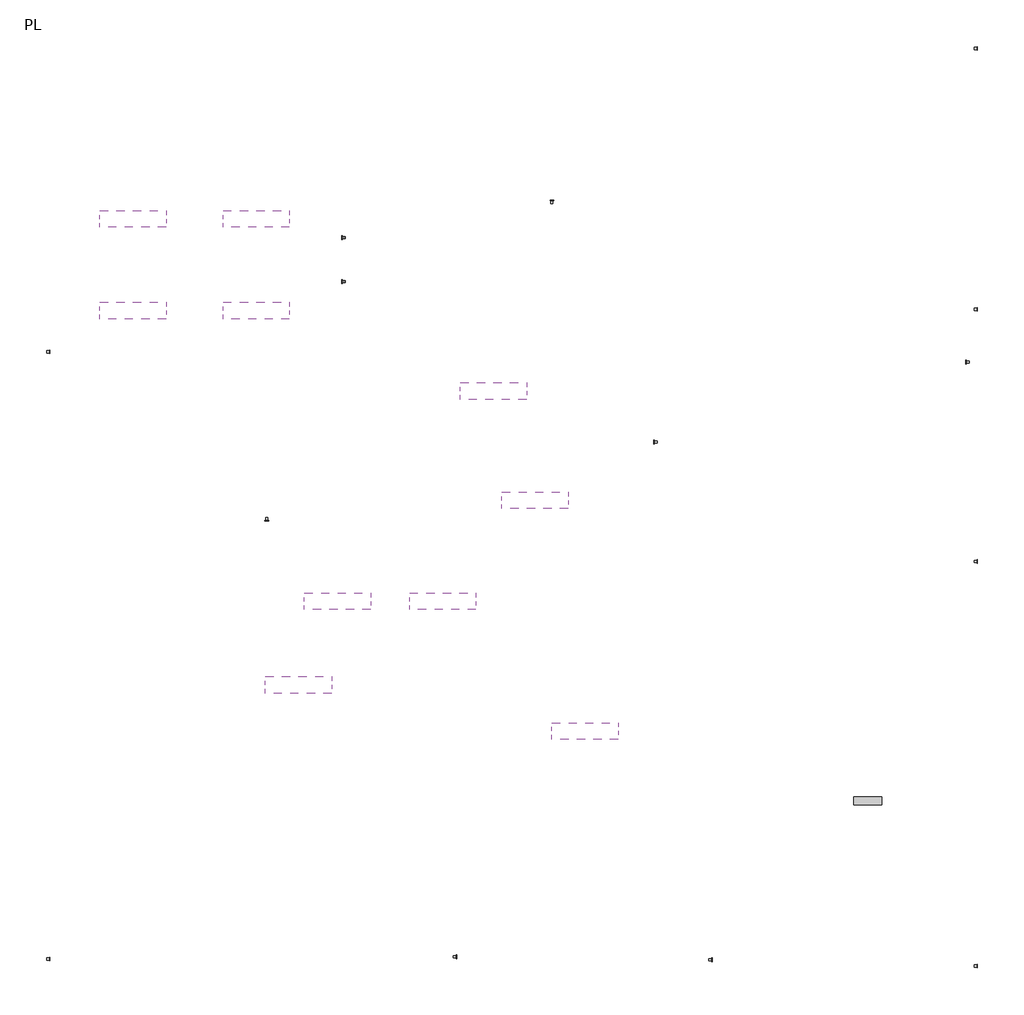
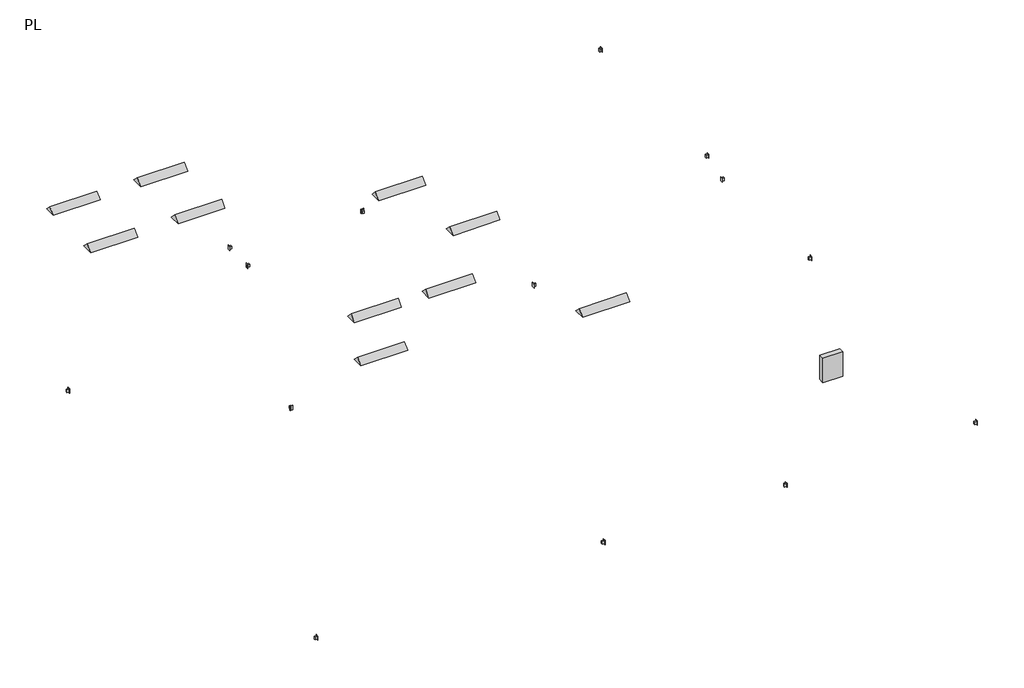
# One storey: 13 proxies, 10 light fixtures, 2 switching devices.
"""IFC4 building model written with IfcOpenShell, lengths in millimetres."""

import ifcopenshell
import ifcopenshell.guid

model = None  # the IFC model being written
_history = None  # IfcOwnerHistory: only IFC2X3 demands one
_inside = {}  # id of a spatial element -> (the spatial element, [elements in it])
_under = {}  # id of a project, library or spatial element -> (it, [spatial elements below it])
_declared = {}  # id of a project -> (the project, [libraries it declares])
_typed = {}  # id of a type object -> (the type object, [elements of that type])
_made_of = {}  # id of a material, layer set ... -> (it, [elements and type objects made of it])


def new_model(schema):
    """Start an empty IFC model of exactly this schema.

    Asked for "IFC4X3", IfcOpenShell would pick the latest addendum, in which some entities
    have other attributes; the version numbers below select the first issue.
    IFC2X3 requires an IfcOwnerHistory on every rooted entity: one is made here for all.
    """
    global model, _history
    if schema == "IFC4X3":
        model = ifcopenshell.file(schema_version=(4, 3, 0, 0))
    else:
        model = ifcopenshell.file(schema=schema)
    _inside.clear()
    _under.clear()
    _declared.clear()
    _typed.clear()
    _made_of.clear()
    _history = None
    if model.schema == "IFC2X3":
        org = make("IfcOrganization", Name="unknown")
        user = make(
            "IfcPersonAndOrganization",
            ThePerson=make("IfcPerson", FamilyName="unknown"),
            TheOrganization=org,
        )
        app = make(
            "IfcApplication",
            ApplicationDeveloper=org,
            Version="unknown",
            ApplicationFullName="unknown",
            ApplicationIdentifier="unknown",
        )
        _history = make(
            "IfcOwnerHistory",
            OwningUser=user,
            OwningApplication=app,
            ChangeAction="ADDED",
            CreationDate=0,
        )
    return model


def make(cls, **values):
    """One entity of the class cls with the attributes given. An attribute that is None is left unset."""
    return model.create_entity(
        cls, **{name: value for name, value in values.items() if value is not None}
    )


def rooted(cls, **values):
    """An entity with a GlobalId (a new one), such as an element, a storey or a relation."""
    return make(cls, GlobalId=ifcopenshell.guid.new(), OwnerHistory=_history, **values)


def si_unit(unit_type, name, prefix=None):
    """IfcSIUnit, for example si_unit("LENGTHUNIT", "METRE", prefix="MILLI")."""
    return make("IfcSIUnit", UnitType=unit_type, Prefix=prefix, Name=name)


def assignment(units):
    """IfcUnitAssignment: the units of a project."""
    return None if units is None else make("IfcUnitAssignment", Units=units)


def point(xyz):
    """IfcCartesianPoint."""
    return None if xyz is None else make("IfcCartesianPoint", Coordinates=xyz)


def direction(xyz):
    """IfcDirection."""
    return None if xyz is None else make("IfcDirection", DirectionRatios=xyz)


def frame(location, z_axis=None, x_axis=None):
    """IfcAxis2Placement3D, a coordinate frame: its origin and axes. An axis left out is left unset."""
    return make(
        "IfcAxis2Placement3D",
        Location=point(location),
        Axis=direction(z_axis),
        RefDirection=direction(x_axis),
    )


def origin():
    """The frame at (0, 0, 0) with its axes left unset."""
    return frame((0.0, 0.0, 0.0))


def origin_with_axes():
    """The frame at (0, 0, 0) with the z axis (0, 0, 1) and the x axis (1, 0, 0) written out."""
    return frame((0.0, 0.0, 0.0), z_axis=(0.0, 0.0, 1.0), x_axis=(1.0, 0.0, 0.0))


def place(relative_to, where):
    """IfcLocalPlacement: puts the frame where relative to a parent placement (None: the world)."""
    return make(
        "IfcLocalPlacement", PlacementRelTo=relative_to, RelativePlacement=where
    )


def context(
    kind, dimensions, precision=None, world=None, true_north=None, identifier=None
):
    """IfcGeometricRepresentationContext, for example the 3D "Model" context."""
    return make(
        "IfcGeometricRepresentationContext",
        ContextIdentifier=identifier,
        ContextType=kind,
        CoordinateSpaceDimension=dimensions,
        Precision=precision,
        WorldCoordinateSystem=world,
        TrueNorth=true_north,
    )


def project(units=None, contexts=None):
    """IfcProject with its units and contexts."""
    return rooted(
        "IfcProject",
        Name="project",
        RepresentationContexts=contexts,
        UnitsInContext=assignment(units),
    )


def spatial(cls, under=None, at=None, **own):
    """A site, building, storey or space (cls), placed at a placement, below another one or the project."""
    s = rooted(cls, ObjectPlacement=at, **own)
    if under is not None:
        _under.setdefault(under.id(), (under, []))[1].append(s)
    return s


def polyline(points):
    """IfcPolyline through the points."""
    return make("IfcPolyline", Points=[point(p) for p in points])


def outline(outer, holes=None, kind="AREA"):
    """IfcArbitraryClosedProfileDef: a profile drawn as a closed curve; with holes, ...WithVoids."""
    if holes is None:
        return make("IfcArbitraryClosedProfileDef", ProfileType=kind, OuterCurve=outer)
    return make(
        "IfcArbitraryProfileDefWithVoids",
        ProfileType=kind,
        OuterCurve=outer,
        InnerCurves=holes,
    )


def extrude(swept, where, along, depth):
    """IfcExtrudedAreaSolid: the profile swept, set in the frame where, extruded along a direction by depth."""
    return make(
        "IfcExtrudedAreaSolid",
        SweptArea=swept,
        Position=where,
        ExtrudedDirection=direction(along),
        Depth=depth,
    )


def shape(context_of_items, identifier, shape_type, items):
    """IfcShapeRepresentation: the items that make up one representation, for example the "Body"."""
    return make(
        "IfcShapeRepresentation",
        ContextOfItems=context_of_items,
        RepresentationIdentifier=identifier,
        RepresentationType=shape_type,
        Items=items,
    )


def source(mapping_origin, context_of_items, identifier, shape_type, items):
    """IfcRepresentationMap: a shape defined once, which mapped items show again and again."""
    return make(
        "IfcRepresentationMap",
        MappingOrigin=mapping_origin,
        MappedRepresentation=shape(context_of_items, identifier, shape_type, items),
    )


def transform(
    local_origin,
    x_axis=None,
    y_axis=None,
    z_axis=None,
    scale=None,
    scale2=None,
    scale3=None,
    uniform=True,
):
    """IfcCartesianTransformationOperator3D, or its non-uniform kind. x_axis, y_axis, z_axis: its Axis1, 2, 3."""
    if uniform:
        return make(
            "IfcCartesianTransformationOperator3D",
            Axis1=direction(x_axis),
            Axis2=direction(y_axis),
            LocalOrigin=point(local_origin),
            Scale=scale,
            Axis3=direction(z_axis),
        )
    return make(
        "IfcCartesianTransformationOperator3DnonUniform",
        Axis1=direction(x_axis),
        Axis2=direction(y_axis),
        LocalOrigin=point(local_origin),
        Scale=scale,
        Axis3=direction(z_axis),
        Scale2=scale2,
        Scale3=scale3,
    )


def mapped(mapping_source, mapping_target):
    """IfcMappedItem: shows the shape of a source again, moved by a transform."""
    return make(
        "IfcMappedItem", MappingSource=mapping_source, MappingTarget=mapping_target
    )


def made_of(thing, what):
    """Note that an element or type object is made of a material, layer set ...; save() writes the relation."""
    if what is not None:
        _made_of.setdefault(what.id(), (what, []))[1].append(thing)
    return thing


def element(
    cls,
    number,
    at=None,
    inside=None,
    cuts=None,
    type_object=None,
    material=None,
    context=None,
    identifier="Body",
    shape_type=None,
    held_by="IfcProductDefinitionShape",
    body=None,
    shapes=None,
    **own,
):
    """One element of the class cls, such as IfcWall. Its Tag is "e" and its number.

    at: its placement. inside: the storey or other place that contains it. cuts: it is an
    opening in that element (IfcRelVoidsElement). A single representation is given by context,
    identifier, shape_type and body (its items); several are given by shapes. held_by: the class
    of the entity that holds the representations. save() writes the other relations.
    """
    e = rooted(cls, Tag="e%d" % number, ObjectPlacement=at, **own)
    if body is not None:
        shapes = [shape(context, identifier, shape_type, body)]
    if shapes is not None:
        e.Representation = make(held_by, Representations=shapes)
    if inside is not None:
        _inside.setdefault(inside.id(), (inside, []))[1].append(e)
    if cuts is not None:
        rooted(
            "IfcRelVoidsElement", RelatingBuildingElement=cuts, RelatedOpeningElement=e
        )
    if type_object is not None:
        _typed.setdefault(type_object.id(), (type_object, []))[1].append(e)
    return made_of(e, material)


def aggregate(whole, parts):
    """IfcRelAggregates: a whole, such as a stair, and the parts it consists of."""
    return rooted("IfcRelAggregates", RelatingObject=whole, RelatedObjects=parts)


def save(model, path):
    """Write the relations noted so far, then the file.

    IfcRelAggregates (storeys below a building ...), IfcRelContainedInSpatialStructure (elements
    in a storey), IfcRelDefinesByType, IfcRelAssociatesMaterial and IfcRelDeclares: one each for
    every whole, place, type object, material and project.
    """
    for whole, parts in _under.values():
        aggregate(whole, parts)
    for where, things in _inside.values():
        rooted(
            "IfcRelContainedInSpatialStructure",
            RelatedElements=things,
            RelatingStructure=where,
        )
    for kind, things in _typed.values():
        rooted("IfcRelDefinesByType", RelatedObjects=things, RelatingType=kind)
    for what, things in _made_of.values():
        rooted("IfcRelAssociatesMaterial", RelatedObjects=things, RelatingMaterial=what)
    for by, libraries in _declared.values():
        rooted("IfcRelDeclares", RelatingContext=by, RelatedDefinitions=libraries)
    model.write(path)


def m_duplex_receptacle_standard_10251bba(model_context):
    return source(origin(), model_context, "Body", "SweptSolid", [
        extrude(outline(polyline([(19.05, 38.1), (19.05, -38.1), (-19.05, -38.1), (-19.05, 38.1), (19.05, 38.1)])), frame((0.0, 0.0, -53.975), z_axis=(0.0, 0.0, 1.0), x_axis=(1.0, 0.0, 0.0)), (0.0, 0.0, 1.0), 53.975),
        extrude(outline(polyline([(34.925, 57.15), (34.925, -57.15), (-34.925, -57.15), (-34.925, 57.15), (34.925, 57.15)])), origin_with_axes(), (0.0, 0.0, 1.0), 4.7625),
    ])


def m_lighting_and_appliance_panelboard_208v_mcb_100_a_975063b2(model_context):
    return source(origin(), model_context, "Body", "SweptSolid", [
        extrude(outline(polyline([(349.2594706, 94.0943297), (349.2594706, -566.3056703), (-158.7405294, -566.3056703), (-158.7405294, 94.0943297), (349.2594706, 94.0943297)])), frame((0.0, 0.0, -146.1), z_axis=(0.0, 0.0, 1.0), x_axis=(1.0, 0.0, 0.0)), (0.0, 0.0, 1.0), 146.1),
    ])


def m_plain_recessed_lighting_fixture_300x1200_120_e46e8774(model_context):
    return source(origin(), model_context, "Body", "SweptSolid", [
        extrude(outline(polyline([(-300.0, 0.0), (0.0, 0.0), (-150.0, -150.0), (-300.0, 0.0)])), frame((0.0, 0.0, 0.0), z_axis=(1.0, 0.0, 0.0), x_axis=(0.0, 1.0, 0.0)), (0.0, 0.0, 1.0), 1200.0),
    ])


model = new_model("IFC4")

# Units and contexts
model_context = context("Model", 3, world=origin())
ifc_project = project(units=[si_unit("LENGTHUNIT", "METRE", prefix="MILLI")], contexts=[model_context])

# Site, building, storey
site = spatial("IfcSite", under=ifc_project)
building = spatial("IfcBuilding", under=site)
storey = spatial("IfcBuildingStorey", under=building, Name="PL", Elevation=500.0)

# Proxies
placement = place(None, origin())
m_duplex_receptacle_standard_shape = m_duplex_receptacle_standard_10251bba(model_context)
element("IfcBuildingElementProxy", 1, Name="M_Duplex Receptacle : Standard", ObjectType="M_Duplex Receptacle : Standard", at=placement, inside=storey, context=model_context, shape_type="MappedRepresentation", body=[
    mapped(m_duplex_receptacle_standard_shape, transform((-14381.6781998, 2753.1971502, 960.0), x_axis=(0.0, -1.0, 0.0), y_axis=(0.0, 0.0, -1.0), z_axis=(1.0, 0.0, 0.0))),
])
element("IfcBuildingElementProxy", 2, Name="M_Duplex Receptacle : Standard", ObjectType="M_Duplex Receptacle : Standard", at=placement, inside=storey, context=model_context, shape_type="MappedRepresentation", body=[
    mapped(m_duplex_receptacle_standard_shape, transform((-14383.0803925, -8248.8260965, 945.9057387), x_axis=(0.0, -1.0, 0.0), y_axis=(0.0, 0.0, -1.0), z_axis=(1.0, 0.0, 0.0))),
])
element("IfcBuildingElementProxy", 3, Name="M_Duplex Receptacle : Standard", ObjectType="M_Duplex Receptacle : Standard", at=placement, inside=storey, context=model_context, shape_type="MappedRepresentation", body=[
    mapped(m_duplex_receptacle_standard_shape, transform((-7014.1011176, -8210.0342024, 931.5557962), x_axis=(0.0, -1.0, 0.0), y_axis=(0.0, 0.0, -1.0), z_axis=(1.0, 0.0, 0.0))),
])
element("IfcBuildingElementProxy", 4, Name="M_Duplex Receptacle : Standard", ObjectType="M_Duplex Receptacle : Standard", at=placement, inside=storey, context=model_context, shape_type="MappedRepresentation", body=[
    mapped(m_duplex_receptacle_standard_shape, transform((-2388.319764, -8264.9137548, 893.2417419), x_axis=(0.0, -1.0, 0.0), y_axis=(0.0, 0.0, -1.0), z_axis=(1.0, 0.0, 0.0))),
])
element("IfcBuildingElementProxy", 5, Name="M_Duplex Receptacle : Standard", ObjectType="M_Duplex Receptacle : Standard", at=placement, inside=storey, context=model_context, shape_type="MappedRepresentation", body=[
    mapped(m_duplex_receptacle_standard_shape, transform((2418.3218002, -8376.2820475, 960.0), x_axis=(0.0, -1.0, 0.0), y_axis=(0.0, 0.0, -1.0), z_axis=(1.0, 0.0, 0.0))),
])
element("IfcBuildingElementProxy", 6, Name="M_Duplex Receptacle : Standard", ObjectType="M_Duplex Receptacle : Standard", at=placement, inside=storey, context=model_context, shape_type="MappedRepresentation", body=[
    mapped(m_duplex_receptacle_standard_shape, transform((2418.3218002, -1043.6002542, 960.0), x_axis=(0.0, -1.0, 0.0), y_axis=(0.0, 0.0, -1.0), z_axis=(1.0, 0.0, 0.0))),
])
element("IfcBuildingElementProxy", 7, Name="M_Duplex Receptacle : Standard", ObjectType="M_Duplex Receptacle : Standard", at=placement, inside=storey, context=model_context, shape_type="MappedRepresentation", body=[
    mapped(m_duplex_receptacle_standard_shape, transform((2418.3218002, 3524.2201594, 960.0), x_axis=(0.0, -1.0, 0.0), y_axis=(0.0, 0.0, -1.0), z_axis=(1.0, 0.0, 0.0))),
])
element("IfcBuildingElementProxy", 8, Name="M_Duplex Receptacle : Standard", ObjectType="M_Duplex Receptacle : Standard", at=placement, inside=storey, context=model_context, shape_type="MappedRepresentation", body=[
    mapped(m_duplex_receptacle_standard_shape, transform((2418.3218002, 8251.436308, 960.0), x_axis=(0.0, -1.0, 0.0), y_axis=(0.0, 0.0, -1.0), z_axis=(1.0, 0.0, 0.0))),
])
element("IfcBuildingElementProxy", 9, Name="M_Duplex Receptacle : Standard", ObjectType="M_Duplex Receptacle : Standard", at=placement, inside=storey, context=model_context, shape_type="MappedRepresentation", body=[
    mapped(m_duplex_receptacle_standard_shape, transform((2218.3218002, 2571.4479124, 960.0), x_axis=(0.0, 1.0, 0.0), y_axis=(0.0, 0.0, -1.0), z_axis=(-1.0, 0.0, 0.0))),
])
element("IfcBuildingElementProxy", 10, Name="M_Duplex Receptacle : Standard", ObjectType="M_Duplex Receptacle : Standard", at=placement, inside=storey, context=model_context, shape_type="MappedRepresentation", body=[
    mapped(m_duplex_receptacle_standard_shape, transform((-5283.4743656, 5494.1412672, 960.0), x_axis=(1.0, 0.0, 0.0), y_axis=(0.0, 0.0, -1.0), z_axis=(0.0, 1.0, 0.0))),
])
element("IfcBuildingElementProxy", 11, Name="M_Duplex Receptacle : Standard", ObjectType="M_Duplex Receptacle : Standard", at=placement, inside=storey, context=model_context, shape_type="MappedRepresentation", body=[
    mapped(m_duplex_receptacle_standard_shape, transform((-10450.4315513, -305.8587328, 960.0), x_axis=(-1.0, 0.0, 0.0), y_axis=(0.0, 0.0, -1.0), z_axis=(0.0, -1.0, 0.0))),
])
element("IfcBuildingElementProxy", 12, Name="M_Duplex Receptacle : Standard", ObjectType="M_Duplex Receptacle : Standard", at=placement, inside=storey, context=model_context, shape_type="MappedRepresentation", body=[
    mapped(m_duplex_receptacle_standard_shape, transform((-3431.6781998, 1122.565095, 960.0), x_axis=(0.0, 1.0, 0.0), y_axis=(0.0, 0.0, -1.0), z_axis=(-1.0, 0.0, 0.0))),
])
m_lighting_and_appliance_panelboard_208v_mcb_100_a_shape = m_lighting_and_appliance_panelboard_208v_mcb_100_a_975063b2(model_context)
element("IfcBuildingElementProxy", 13, Name="M_Lighting and Appliance Panelboard - 208V MCB : 100 A", ObjectType="M_Lighting and Appliance Panelboard - 208V MCB : 100 A", at=placement, inside=storey, context=model_context, shape_type="MappedRepresentation", body=[
    mapped(m_lighting_and_appliance_panelboard_208v_mcb_100_a_shape, transform((337.9433717, -5451.9587328, 1605.9056703), x_axis=(1.0, 0.0, 0.0), y_axis=(0.0, 0.0, 1.0), z_axis=(0.0, -1.0, 0.0))),
])

# Light fixtures
m_plain_recessed_lighting_fixture_300x1200_120_shape = m_plain_recessed_lighting_fixture_300x1200_120_e46e8774(model_context)
element("IfcLightFixture", 14, ObjectType="M_Plain Recessed Lighting Fixture : 300x1200 - 120", at=placement, inside=storey, context=model_context, shape_type="MappedRepresentation", body=[
    mapped(m_plain_recessed_lighting_fixture_300x1200_120_shape, transform((-13471.5716878, 3351.0879554, 4000.0), x_axis=(1.0, 0.0, 0.0), y_axis=(0.0, -1.0, 0.0), z_axis=(0.0, 0.0, -1.0))),
])
element("IfcLightFixture", 15, ObjectType="M_Plain Recessed Lighting Fixture : 300x1200 - 120", at=placement, inside=storey, context=model_context, shape_type="MappedRepresentation", body=[
    mapped(m_plain_recessed_lighting_fixture_300x1200_120_shape, transform((-13471.5716878, 5008.8069678, 4000.0), x_axis=(1.0, 0.0, 0.0), y_axis=(0.0, -1.0, 0.0), z_axis=(0.0, 0.0, -1.0))),
])
element("IfcLightFixture", 16, ObjectType="M_Plain Recessed Lighting Fixture : 300x1200 - 120", at=placement, inside=storey, context=model_context, shape_type="MappedRepresentation", body=[
    mapped(m_plain_recessed_lighting_fixture_300x1200_120_shape, transform((-11238.106009, 5008.8069678, 4000.0), x_axis=(1.0, 0.0, 0.0), y_axis=(0.0, -1.0, 0.0), z_axis=(0.0, 0.0, -1.0))),
])
element("IfcLightFixture", 17, ObjectType="M_Plain Recessed Lighting Fixture : 300x1200 - 120", at=placement, inside=storey, context=model_context, shape_type="MappedRepresentation", body=[
    mapped(m_plain_recessed_lighting_fixture_300x1200_120_shape, transform((-11238.106009, 3351.0879554, 4000.0), x_axis=(1.0, 0.0, 0.0), y_axis=(0.0, -1.0, 0.0), z_axis=(0.0, 0.0, -1.0))),
])
element("IfcLightFixture", 18, ObjectType="M_Plain Recessed Lighting Fixture : 300x1200 - 120", at=placement, inside=storey, context=model_context, shape_type="MappedRepresentation", body=[
    mapped(m_plain_recessed_lighting_fixture_300x1200_120_shape, transform((-10474.940669, -3432.5980118, 4000.0), x_axis=(1.0, 0.0, 0.0), y_axis=(0.0, -1.0, 0.0), z_axis=(0.0, 0.0, -1.0))),
])
element("IfcLightFixture", 19, ObjectType="M_Plain Recessed Lighting Fixture : 300x1200 - 120", at=placement, inside=storey, context=model_context, shape_type="MappedRepresentation", body=[
    mapped(m_plain_recessed_lighting_fixture_300x1200_120_shape, transform((-5283.4493688, -4265.8003192, 4000.0), x_axis=(1.0, 0.0, 0.0), y_axis=(0.0, -1.0, 0.0), z_axis=(0.0, 0.0, -1.0))),
])
element("IfcLightFixture", 20, ObjectType="M_Plain Recessed Lighting Fixture : 300x1200 - 120", at=placement, inside=storey, context=model_context, shape_type="MappedRepresentation", body=[
    mapped(m_plain_recessed_lighting_fixture_300x1200_120_shape, transform((-6188.4168093, -89.5432203, 4000.0), x_axis=(1.0, 0.0, 0.0), y_axis=(0.0, -1.0, 0.0), z_axis=(0.0, 0.0, -1.0))),
])
element("IfcLightFixture", 21, ObjectType="M_Plain Recessed Lighting Fixture : 300x1200 - 120", at=placement, inside=storey, context=model_context, shape_type="MappedRepresentation", body=[
    mapped(m_plain_recessed_lighting_fixture_300x1200_120_shape, transform((-6944.285007, 1892.7111009, 4000.0), x_axis=(1.0, 0.0, 0.0), y_axis=(0.0, -1.0, 0.0), z_axis=(0.0, 0.0, -1.0))),
])
element("IfcLightFixture", 22, ObjectType="M_Plain Recessed Lighting Fixture : 300x1200 - 120", at=placement, inside=storey, context=model_context, shape_type="MappedRepresentation", body=[
    mapped(m_plain_recessed_lighting_fixture_300x1200_120_shape, transform((-7860.4121676, -1918.3778872, 4000.0), x_axis=(1.0, 0.0, 0.0), y_axis=(0.0, -1.0, 0.0), z_axis=(0.0, 0.0, -1.0))),
])
element("IfcLightFixture", 23, ObjectType="M_Plain Recessed Lighting Fixture : 300x1200 - 120", at=placement, inside=storey, context=model_context, shape_type="MappedRepresentation", body=[
    mapped(m_plain_recessed_lighting_fixture_300x1200_120_shape, transform((-9765.9566616, -1918.3778872, 4000.0), x_axis=(1.0, 0.0, 0.0), y_axis=(0.0, -1.0, 0.0), z_axis=(0.0, 0.0, -1.0))),
])

# Switching devices
element("IfcSwitchingDevice", 24, ObjectType="M_Lighting Switches : Three Way", at=placement, inside=storey, context=model_context, shape_type="MappedRepresentation", body=[
    mapped(m_duplex_receptacle_standard_shape, transform((-9081.6781998, 4824.0225299, 1700.0), x_axis=(0.0, -1.0, 0.0), y_axis=(0.0, 0.0, 1.0), z_axis=(-1.0, 0.0, 0.0))),
])
element("IfcSwitchingDevice", 25, ObjectType="M_Lighting Switches : Three Way", at=placement, inside=storey, context=model_context, shape_type="MappedRepresentation", body=[
    mapped(m_duplex_receptacle_standard_shape, transform((-9081.6781998, 4027.3902163, 1700.0), x_axis=(0.0, -1.0, 0.0), y_axis=(0.0, 0.0, 1.0), z_axis=(-1.0, 0.0, 0.0))),
])

save(model, "model.ifc")

# Revit data of these elements
# Project information
#   Project Issue Date = "Issue Date"
#   Project Status = "Project Status"
#   Client Name = "Owner"
#   Project Address = "Enter address here"
#   Project Name = "Project Name"
#   Project Number = "Project Number"
# Type "M_Duplex Receptacle : Standard"
#   Label = ""
#   Switch Voltage = 120 V
#   Load = 180 VA
#   Default Elevation = 460 mm
#   Load Classification = Receptacle
#   Assembly Code = ""
# Type "M_Lighting and Appliance Panelboard - 208V MCB : 100 A"
#   built-in parameter 1140081 [instance default] = "Recessed"
#   built-in parameter 1140083 [instance default] = "Type 1"
#   Width = 508 mm
#   built-in parameter 1140082 [instance default] = 100 (stored number, unit not read)
#   built-in parameter 1140140 = 100 (stored number, unit not read)
#   Height [instance default] = 584.2 mm
#   Depth = 146.1 mm
#   Default Elevation = 1200 mm
#   42 Circuit Height = 1270 mm
#   30 Circuit Height = 736.6 mm
#   24 Circuit Height = 660.4 mm
#   12 Circuit Height = 584.2 mm
#   built-in parameter 1140079 [instance default] = 12
#   Load Classification = Other
# Type "M_Plain Recessed Lighting Fixture : 300x1200 - 120"
#   Photometric Web File = "1x42A12.ies"
#   Width = 300 mm
#   Wattage = 64 W
#   built-in parameter 1150110 = 1 (stored number, unit not read)
#   built-in parameter 1150109 = 1 (stored number, unit not read)
#   built-in parameter 1150113 = 1 (stored number, unit not read)
#   Tilt Angle = -90.00°
#   Lumens = 5699.84 lm
#   built-in parameter 1114217 = 0.88 (stored number, unit not read)
#   built-in parameter 1150115 = 1 (stored number, unit not read)
#   built-in parameter 1150105 = 453.579 (stored number, unit not read)
#   Length = 1200 mm
#   built-in parameter 1150112 = 1 (stored number, unit not read)
#   built-in parameter 1150114 = 1 (stored number, unit not read)
#   built-in parameter 1150107 = 4230 (stored number, unit not read)
#   built-in parameter 1150106 = 4.53579 (stored number, unit not read)
#   Emit from Rectangle Width = 300 mm
#   Emit from Rectangle Length = 1200 mm
#   built-in parameter 1150104 = 8.27394 (stored number, unit not read)
#   Depth = 150 mm
#   Default Elevation = 2000 mm
#   Ballast Voltage = 120 V
#   built-in parameter 1114218 = 0.88 (stored number, unit not read)
#   built-in parameter 1150133 = 10 (stored number, unit not read)
#   Apparent Load = 64 VA
#   built-in parameter 1150134 = 8
#   built-in parameter 1150137 = 1
#   Color Filter = 16777215
#   built-in parameter 1140040 [instance default] = 1
#   Load Classification = Lighting - Dwelling Unit
#   Emit Shape Visible in Rendering = no
#   Dimming Lamp Color Temperature Shift = (empty or 0)
#   Assembly Code = ""
# Type "M_Lighting Switches : Three Way"
#   Label = "3"
#   Switch Voltage [instance default] = 120 V
#   Default Elevation = 1200 mm
#   Apparent Load = 0 VA
#   Load Classification = Other
#   Assembly Code = ""
# Element 1 (IfcBuildingElementProxy, "M_Duplex Receptacle : Standard")
#   Mark = "1"
#   Phase Created = New Construction
# Element 2 (IfcBuildingElementProxy, "M_Duplex Receptacle : Standard")
#   Mark = "2"
#   Phase Created = New Construction
# Element 3 (IfcBuildingElementProxy, "M_Duplex Receptacle : Standard")
#   Mark = "3"
#   Phase Created = New Construction
# Element 4 (IfcBuildingElementProxy, "M_Duplex Receptacle : Standard")
#   Mark = "4"
#   Phase Created = New Construction
# Element 5 (IfcBuildingElementProxy, "M_Duplex Receptacle : Standard")
#   Mark = "5"
#   Phase Created = New Construction
# Element 6 (IfcBuildingElementProxy, "M_Duplex Receptacle : Standard")
#   Mark = "6"
#   Phase Created = New Construction
# Element 7 (IfcBuildingElementProxy, "M_Duplex Receptacle : Standard")
#   Mark = "7"
#   Phase Created = New Construction
# Element 8 (IfcBuildingElementProxy, "M_Duplex Receptacle : Standard")
#   Mark = "8"
#   Phase Created = New Construction
# Element 9 (IfcBuildingElementProxy, "M_Duplex Receptacle : Standard")
#   Mark = "9"
#   Phase Created = New Construction
# Element 10 (IfcBuildingElementProxy, "M_Duplex Receptacle : Standard")
#   Mark = "10"
#   Phase Created = New Construction
# Element 11 (IfcBuildingElementProxy, "M_Duplex Receptacle : Standard")
#   Mark = "11"
#   Phase Created = New Construction
# Element 12 (IfcBuildingElementProxy, "M_Duplex Receptacle : Standard")
#   Mark = "12"
#   Phase Created = New Construction
# Element 13 (IfcBuildingElementProxy, "M_Lighting and Appliance Panelboard - 208V MCB : 100 A")
#   Mark = "4"
#   built-in parameter 1140081 = "Recessed"
#   built-in parameter 1140083 = "Type 1"
#   built-in parameter 1140082 = 100 (stored number, unit not read)
#   Height = 660.4 mm
#   built-in parameter 1140079 = 20
#   built-in parameter 1140064 = 120/208 Wye
#   Phase Created = New Construction
# Element 14 (IfcLightFixture, "M_Plain Recessed Lighting Fixture : 300x1200 - 120")
#   Mark = "1"
#   built-in parameter 1140040 = 1
#   Phase Created = New Construction
# Element 15 (IfcLightFixture, "M_Plain Recessed Lighting Fixture : 300x1200 - 120")
#   Mark = "2"
#   built-in parameter 1140040 = 1
#   Phase Created = New Construction
# Element 16 (IfcLightFixture, "M_Plain Recessed Lighting Fixture : 300x1200 - 120")
#   Mark = "3"
#   built-in parameter 1140040 = 1
#   Phase Created = New Construction
# Element 17 (IfcLightFixture, "M_Plain Recessed Lighting Fixture : 300x1200 - 120")
#   Mark = "4"
#   built-in parameter 1140040 = 1
#   Phase Created = New Construction
# Element 18 (IfcLightFixture, "M_Plain Recessed Lighting Fixture : 300x1200 - 120")
#   Mark = "5"
#   built-in parameter 1140040 = 1
#   Phase Created = New Construction
# Element 19 (IfcLightFixture, "M_Plain Recessed Lighting Fixture : 300x1200 - 120")
#   Mark = "7"
#   built-in parameter 1140040 = 1
#   Phase Created = New Construction
# Element 20 (IfcLightFixture, "M_Plain Recessed Lighting Fixture : 300x1200 - 120")
#   Mark = "8"
#   built-in parameter 1140040 = 1
#   Phase Created = New Construction
# Element 21 (IfcLightFixture, "M_Plain Recessed Lighting Fixture : 300x1200 - 120")
#   Mark = "9"
#   built-in parameter 1140040 = 1
#   Phase Created = New Construction
# Element 22 (IfcLightFixture, "M_Plain Recessed Lighting Fixture : 300x1200 - 120")
#   Mark = "10"
#   built-in parameter 1140040 = 1
#   Phase Created = New Construction
# Element 23 (IfcLightFixture, "M_Plain Recessed Lighting Fixture : 300x1200 - 120")
#   Mark = "11"
#   built-in parameter 1140040 = 1
#   Phase Created = New Construction
# Element 24 (IfcSwitchingDevice, "M_Lighting Switches : Three Way")
#   Mark = "1"
#   Switch Voltage = 120 V
#   Phase Created = New Construction
# Element 25 (IfcSwitchingDevice, "M_Lighting Switches : Three Way")
#   Mark = "2"
#   Switch Voltage = 120 V
#   Phase Created = New Construction
